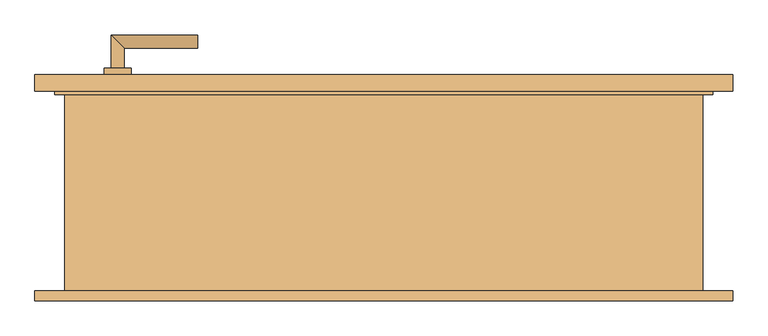
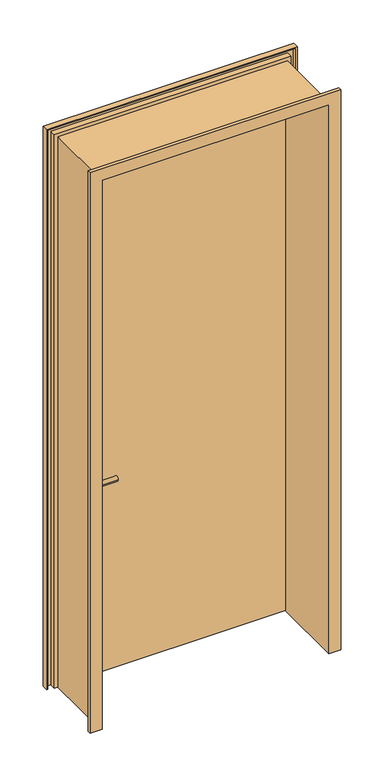
"""IFC4 building model written with IfcOpenShell, lengths in millimetres: door geometry, Drehflügel 1-flg - Stahlzarge : Holztüre 1,0 x 2,45."""

from ifc_helpers import new_model, si_unit, point, frame, frame_2d, origin, place, context, project, spatial, polyline, circle_curve, ellipse_curve, trimmed, segment, composite_curve, outline, extrude, faceted_brep, source, transform, mapped, element, save
from ifc_brep_helpers import plane_surface, cylinder_surface, advanced_brep


def door_89f0df96(model_context):
    return source(origin(), model_context, "Body", "SolidModel", [
        advanced_brep(
        [(-410.0, 139.4346141, 1000.0), (-390.0, 139.4346141, 1000.0), (-410.0, 69.4346141, 1000.0), (-390.0, 89.4346141, 1000.0), (-280.0, 69.4346141, 1000.0), (-280.0, 89.4346141, 1000.0)],
        [
            (0, 1, circle_curve(frame((-400.0, 139.4346141, 1000.0), z_axis=(0.0, 1.0, 0.0), x_axis=(1.0, 0.0, 0.0)), 10.0)),
            (1, 0, circle_curve(frame((-400.0, 139.4346141, 1000.0), z_axis=(0.0, 1.0, 0.0), x_axis=(1.0, 0.0, 0.0)), 10.0)),
            (0, 2),
            (2, 3, ellipse_curve(frame((-400.0, 79.4346141, 1000.0), z_axis=(-0.7071067811865385, 0.7071067811865565, 0.0), x_axis=(0.7071067811865563, 0.7071067811865386, 0.0)), 14.1421356, 10.0)),
            (3, 1),
            (3, 2, ellipse_curve(frame((-400.0, 79.4346141, 1000.0), z_axis=(-0.7071067811865385, 0.7071067811865565, 0.0), x_axis=(0.7071067811865563, 0.7071067811865386, 0.0)), 14.1421356, 10.0)),
            (4, 5, circle_curve(frame((-280.0, 79.4346141, 1000.0), z_axis=(1.0, 0.0, 0.0), x_axis=(0.0, 1.0, 0.0)), 10.0)),
            (5, 4, circle_curve(frame((-280.0, 79.4346141, 1000.0), z_axis=(1.0, 0.0, 0.0), x_axis=(0.0, 1.0, 0.0)), 10.0)),
            (2, 4),
            (5, 3),
        ],
        [
            plane_surface(frame((-400.0, 139.4346141, -287.7526403), z_axis=(0.0, 1.0, 0.0), x_axis=(0.0, 0.0, 1.0))),
            cylinder_surface(frame((-400.0, 139.4346141, 1000.0), z_axis=(0.0, 1.0, 0.0), x_axis=(1.0, 0.0, 0.0)), 10.0),
            plane_surface(frame((-280.0, 79.4346141, -287.7526403), z_axis=(1.0, 0.0, 0.0), x_axis=(0.0, 0.0, 1.0))),
            cylinder_surface(frame((-400.0, 79.4346141, 1000.0), z_axis=(-1.0, 0.0, 0.0), x_axis=(0.0, 1.0, 0.0)), 10.0),
        ],
        [
            (0, [[1, 2]]),
            (1, [[-1, 3, 4, 5]]),
            (1, [[-2, -5, 6, -3]]),
            (2, [[7, 8]]),
            (3, [[-4, 9, -8, 10]]),
            (3, [[-6, -10, -7, -9]]),
        ],
    ),
        advanced_brep(
        [(-390.0, 199.4346141, 1000.0), (-410.0, 199.4346141, 1000.0), (-390.0, 229.4346141, 1000.0), (-410.0, 249.4346141, 1000.0), (-280.0, 229.4346141, 1000.0), (-280.0, 249.4346141, 1000.0)],
        [
            (0, 1, circle_curve(frame((-400.0, 199.4346141, 1000.0), z_axis=(0.0, -1.0, 0.0), x_axis=(-1.0, 0.0, 0.0)), 10.0)),
            (1, 0, circle_curve(frame((-400.0, 199.4346141, 1000.0), z_axis=(0.0, -1.0, 0.0), x_axis=(-1.0, 0.0, 0.0)), 10.0)),
            (0, 2),
            (2, 3, ellipse_curve(frame((-400.0, 239.4346141, 1000.0), z_axis=(-0.7071067811865475, -0.7071067811865475, 0.0), x_axis=(0.7071067811865474, -0.7071067811865476, 0.0)), 14.1421356, 10.0)),
            (3, 1),
            (3, 2, ellipse_curve(frame((-400.0, 239.4346141, 1000.0), z_axis=(-0.7071067811865475, -0.7071067811865475, 0.0), x_axis=(0.7071067811865474, -0.7071067811865476, 0.0)), 14.1421356, 10.0)),
            (4, 5, circle_curve(frame((-280.0, 239.4346141, 1000.0), z_axis=(1.0, 0.0, 0.0), x_axis=(0.0, 1.0, 0.0)), 10.0)),
            (5, 4, circle_curve(frame((-280.0, 239.4346141, 1000.0), z_axis=(1.0, 0.0, 0.0), x_axis=(0.0, 1.0, 0.0)), 10.0)),
            (2, 4),
            (5, 3),
        ],
        [
            plane_surface(frame((-400.0, 199.4346141, -287.7526403), z_axis=(0.0, -1.0, 0.0), x_axis=(0.0, 0.0, 1.0))),
            cylinder_surface(frame((-400.0, 199.4346141, 1000.0), z_axis=(0.0, -1.0, 0.0), x_axis=(-1.0, 0.0, 0.0)), 10.0),
            plane_surface(frame((-280.0, 239.4346141, -287.7526403), z_axis=(1.0, 0.0, 0.0), x_axis=(0.0, 0.0, 1.0))),
            cylinder_surface(frame((-400.0, 239.4346141, 1000.0), z_axis=(-1.0, 0.0, 0.0), x_axis=(0.0, 1.0, 0.0)), 10.0),
        ],
        [
            (0, [[1, 2]]),
            (1, [[-1, 3, 4, 5]]),
            (1, [[-2, -5, 6, -3]]),
            (2, [[7, 8]]),
            (3, [[-4, 9, -8, 10]]),
            (3, [[-6, -10, -7, -9]]),
        ],
    ),
        extrude(outline(composite_curve([segment(trimmed(circle_curve(frame_2d((1000.0, -400.0)), 20.0), [point((1000.0, -420.0))], [point((1000.0, -380.0))], False, "CARTESIAN"), True, "CONTINUOUS"), segment(trimmed(circle_curve(frame_2d((1000.0, -400.0)), 20.0), [point((1000.0, -380.0))], [point((1000.0, -420.0))], False, "CARTESIAN"), True, "CONTINUOUS")], self_intersect=False)), frame((0.0, 129.4346141, 0.0), z_axis=(0.0, 1.0, 0.0), x_axis=(0.0, 0.0, 1.0)), (0.0, 0.0, 1.0), 10.0),
        extrude(outline(composite_curve([segment(trimmed(circle_curve(frame_2d((1000.0, -400.0)), 20.0), [point((1000.0, -420.0))], [point((1000.0, -380.0))], False, "CARTESIAN"), True, "CONTINUOUS"), segment(trimmed(circle_curve(frame_2d((1000.0, -400.0)), 20.0), [point((1000.0, -380.0))], [point((1000.0, -420.0))], False, "CARTESIAN"), True, "CONTINUOUS")], self_intersect=False)), frame((0.0, 189.4346141, 0.0), z_axis=(0.0, 1.0, 0.0), x_axis=(0.0, 0.0, 1.0)), (0.0, 0.0, 1.0), 10.0),
        extrude(outline(polyline([(490.0, 164.4346141), (-490.0, 164.4346141), (-490.0, 189.4346141), (490.0, 189.4346141), (490.0, 164.4346141)])), frame((0.0, 0.0, 100.0), z_axis=(0.0, 0.0, 1.0), x_axis=(1.0, 0.0, 0.0)), (0.0, 0.0, 1.0), 2440.0),
        faceted_brep([(524.4603207, -150.5653859, 100.0), (475.0, -150.5653859, 100.0), (475.0, 164.4346141, 100.0), (490.0, 164.4346141, 100.0), (490.0, 189.4346141, 100.0), (524.4603207, 189.4346141, 100.0), (524.4603207, 164.4346141, 100.0), (519.4603207, 164.4346141, 100.0), (519.4603207, 184.4346141, 100.0), (495.0, 184.4346141, 100.0), (495.0, 159.4346141, 100.0), (480.0, 159.4346141, 100.0), (480.0, -145.5653859, 100.0), (519.4603207, -145.5653859, 100.0), (519.4603207, -135.5653859, 100.0), (524.4603207, -135.5653859, 100.0), (524.4603207, -150.5653859, 2574.4603207), (-524.4603207, -150.5653859, 2574.4603207), (-524.4603207, -150.5653859, 100.0), (-475.0, -150.5653859, 100.0), (-475.0, -150.5653859, 2525.0), (475.0, -150.5653859, 2525.0), (475.0, 164.4346141, 2525.0), (-475.0, 164.4346141, 2525.0), (-475.0, 164.4346141, 100.0), (-490.0, 164.4346141, 100.0), (-490.0, 164.4346141, 2540.0), (490.0, 164.4346141, 2540.0), (490.0, 189.4346141, 2540.0), (-490.0, 189.4346141, 2540.0), (-490.0, 189.4346141, 100.0), (-524.4603207, 189.4346141, 100.0), (-524.4603207, 189.4346141, 2574.4603207), (524.4603207, 189.4346141, 2574.4603207), (524.4603207, 164.4346141, 2574.4603207), (-524.4603207, 164.4346141, 2574.4603207), (-524.4603207, 164.4346141, 100.0), (-519.4603207, 164.4346141, 100.0), (-519.4603207, 164.4346141, 2569.4603207), (519.4603207, 164.4346141, 2569.4603207), (519.4603207, 184.4346141, 2569.4603207), (-519.4603207, 184.4346141, 2569.4603207), (-519.4603207, 184.4346141, 100.0), (-495.0, 184.4346141, 100.0), (-495.0, 184.4346141, 2545.0), (495.0, 184.4346141, 2545.0), (495.0, 159.4346141, 2545.0), (-495.0, 159.4346141, 2545.0), (-495.0, 159.4346141, 100.0), (-480.0, 159.4346141, 100.0), (-480.0, 159.4346141, 2530.0), (480.0, 159.4346141, 2530.0), (480.0, -145.5653859, 2530.0), (-480.0, -145.5653859, 2530.0), (-480.0, -145.5653859, 100.0), (-519.4603207, -145.5653859, 100.0), (-519.4603207, -145.5653859, 2569.4603207), (519.4603207, -145.5653859, 2569.4603207), (519.4603207, -135.5653859, 2569.4603207), (-519.4603207, -135.5653859, 2569.4603207), (-519.4603207, -135.5653859, 100.0), (-524.4603207, -135.5653859, 100.0), (-524.4603207, -135.5653859, 2574.4603207), (524.4603207, -135.5653859, 2574.4603207)], [[[0, 1, 2, 3, 4, 5, 6, 7, 8, 9, 10, 11, 12, 13, 14, 15]], [[1, 0, 16, 17, 18, 19, 20, 21]], [[2, 1, 21, 22]], [[3, 2, 22, 23, 24, 25, 26, 27]], [[4, 3, 27, 28]], [[5, 4, 28, 29, 30, 31, 32, 33]], [[6, 5, 33, 34]], [[7, 6, 34, 35, 36, 37, 38, 39]], [[8, 7, 39, 40]], [[9, 8, 40, 41, 42, 43, 44, 45]], [[10, 9, 45, 46]], [[11, 10, 46, 47, 48, 49, 50, 51]], [[12, 11, 51, 52]], [[13, 12, 52, 53, 54, 55, 56, 57]], [[14, 13, 57, 58]], [[15, 14, 58, 59, 60, 61, 62, 63]], [[0, 15, 63, 16]], [[17, 62, 61, 18]], [[18, 61, 60, 55, 54, 49, 48, 43, 42, 37, 36, 31, 30, 25, 24, 19]], [[23, 20, 19, 24]], [[29, 26, 25, 30]], [[35, 32, 31, 36]], [[41, 38, 37, 42]], [[47, 44, 43, 48]], [[53, 50, 49, 54]], [[59, 56, 55, 60]], [[22, 21, 20, 23]], [[28, 27, 26, 29]], [[34, 33, 32, 35]], [[40, 39, 38, 41]], [[46, 45, 44, 47]], [[52, 51, 50, 53]], [[58, 57, 56, 59]], [[16, 63, 62, 17]]]),
    ])


if __name__ == "__main__":
    model = new_model("IFC4")
    model_context = context("Model", 3, world=origin())
    ifc_project = project(units=[si_unit("LENGTHUNIT", "METRE", prefix="MILLI")], contexts=[model_context])
    site = spatial("IfcSite", under=ifc_project)
    building = spatial("IfcBuilding", under=site)
    placement = place(None, origin())
    door_shape = door_89f0df96(model_context)
    element("IfcDoor", 1, ObjectType="Drehflügel 1-flg - Stahlzarge : Holztüre 1,0 x 2,45", at=placement, inside=building, context=model_context, shape_type="MappedRepresentation", body=[
        mapped(door_shape, transform((0.0, 0.0, 0.0), x_axis=(1.0, 0.0, 0.0), y_axis=(0.0, 1.0, 0.0), z_axis=(0.0, 0.0, 1.0))),
    ])
    save(model, "model.ifc")

# Revit data of these elements
# Type "Drehflügel 1-flg - Stahlzarge : Holztüre 1,0 x 2,45"
#   Type Mark = "23"
#   Operation = "SingleSwingRight"
#   Keynote = "16.03"
#   Analytic Construction = "Metall"
#   Thermal Resistance (R) = 0.270117 (m²·K)/W
#   Heat Transfer Coefficient (U) = 3.7021 W/(m²·K)
#   Rough Width = 1.000 m
#   Rough Height [instance default] = 2.550 m
#   Höhe Türgriff [instance default] = 0.900 m
#   Height = 2.450 m
#   Fußbodenaufbau [instance default] = 0.100 m
#   Width = 1.000 m
#   Sichtbarkeit Sturzlinien [instance default] = yes
#   Türgriff auswählen [instance default] = element 221079
#   Türgriff [instance default] = none
#   Türflügel [instance default] = none
#   Rahmen/Pfosten [instance default] = Metall - Lackiert - Grau
#   Visual Light Transmittance = 0
#   Solar Heat Gain Coefficient = 0
#   Function = (empty or 0)
#   Wall Closure = (empty or 0)
# Element 1 (IfcDoor, "Drehflügel 1-flg - Stahlzarge : Holztüre 1,0 x 2,45")
#   Rahmen/Pfosten = Holz - Eiche
#   Materials on its faces: "Holz - Eiche", "Metall - Chrom", "Holz - Birke"
# Materials
#   "Metall - Lackiert - Grau": class "Farbe 1", colour RGB 98 98 98, transparency 0, Cost = 0
#   "Holz - Eiche": class "Holz", colour RGB 151 89 53, transparency 0, Cost = 0
#   "Metall - Chrom": class "Metall", colour RGB 247 247 247, transparency 0, Cost = 0
#   "Holz - Birke": class "Holz", colour RGB 213 164 103, transparency 0, Cost = 0
